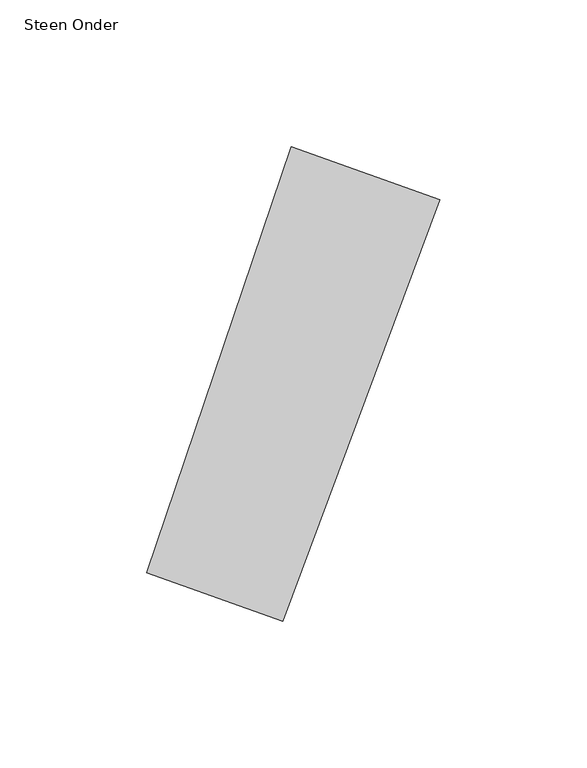
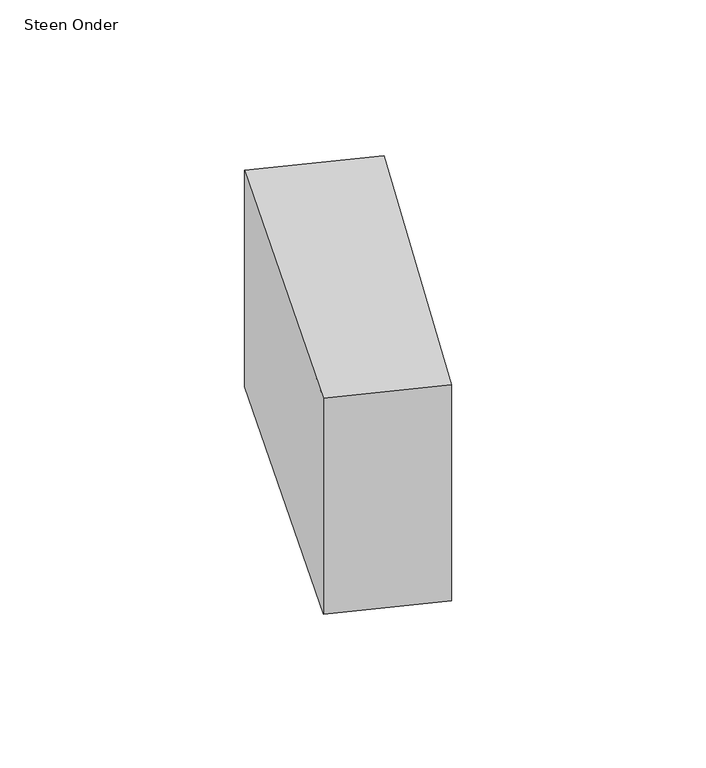
"""IFC4 building model written with IfcOpenShell, lengths in millimetres: proxy geometry, 00_GMA_steen_versie_4 : Steen Onder."""

from ifc_helpers import new_model, si_unit, origin, origin_with_axes, place, context, project, spatial, polyline, outline, extrude, source, transform, mapped, element, save


def steen_onder_dd1e1765(model_context):
    return source(origin(), model_context, "Body", "SweptSolid", [
        extrude(outline(polyline([(126.7746811, 139.9259489), (73.2525302, -3.8273381), (26.8061402, 12.684166), (76.0341035, 157.9640193), (126.7746811, 139.9259489)])), origin_with_axes(), (0.0, 0.0, 1.0), 100.0),
    ])


if __name__ == "__main__":
    model = new_model("IFC4")
    model_context = context("Model", 3, world=origin())
    ifc_project = project(units=[si_unit("LENGTHUNIT", "METRE", prefix="MILLI")], contexts=[model_context])
    site = spatial("IfcSite", under=ifc_project)
    building = spatial("IfcBuilding", under=site)
    placement = place(None, origin())
    steen_onder_shape = steen_onder_dd1e1765(model_context)
    element("IfcBuildingElementProxy", 1, Name="00_GMA_steen_versie_4 : Steen Onder", ObjectType="00_GMA_steen_versie_4 : Steen Onder", at=placement, inside=building, context=model_context, shape_type="MappedRepresentation", body=[
        mapped(steen_onder_shape, transform((0.0, 0.0, 0.0), x_axis=(1.0, 0.0, 0.0), y_axis=(0.0, 1.0, 0.0), z_axis=(0.0, 0.0, 1.0))),
    ])
    save(model, "model.ifc")

# Revit data of these elements
# Type "00_GMA_steen_versie_4 : Steen Onder"
#   StootVoegHalfBoven [instance default] = 5 mm
#   StootVoegHalf [instance default] = 5 mm
#   StootVoegBreedteOnder = 10 mm
#   StootVoegBreedteBoven = 10 mm
#   Steendikte = 100 mm
#   LintVoegOnderHalf = 0 mm
#   LintVoegOnder = 0 mm
#   LintVoegBovenHalf = 5 mm
#   LintVoegBoven = 10 mm
#   materiaal = none
#   MateriaalVoeg = none
#   Default Elevation = 0
